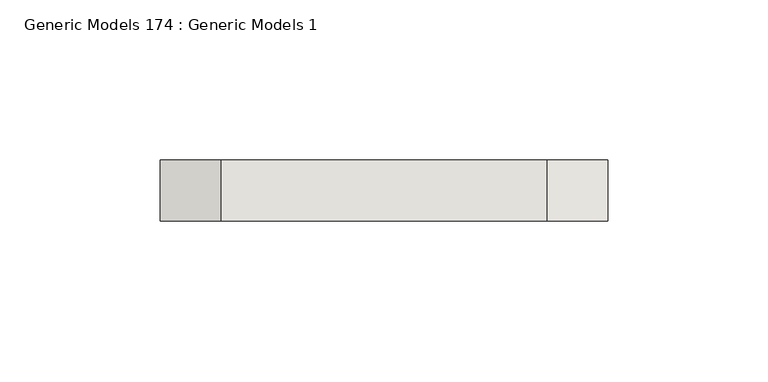
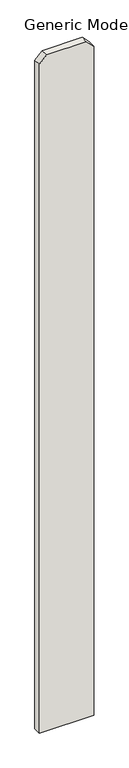
"""IFC4 building model written with IfcOpenShell, lengths in millimetres: wall geometry, Generic Models 174 : Generic Models 1."""

from ifc_helpers import new_model, si_unit, frame, origin, place, context, project, spatial, polyline, outline, extrude, source, transform, mapped, element, save


def generic_models_174_generic_models_1_8f357170(model_context):
    return source(origin(), model_context, "Body", "SweptSolid", [
        extrude(outline(polyline([(76.2, 325499.4125), (1885.95, 325499.4125), (1905.0, 325480.3625), (1905.0, 325378.7625), (1885.95, 325359.7125), (76.2, 325359.7125), (76.2, 325499.4125)])), frame((0.0, 547.6875, 0.0), z_axis=(0.0, 1.0, 0.0), x_axis=(0.0, 0.0, 1.0)), (0.0, 0.0, 1.0), 19.05),
    ])


if __name__ == "__main__":
    model = new_model("IFC4")
    model_context = context("Model", 3, world=origin())
    ifc_project = project(units=[si_unit("LENGTHUNIT", "METRE", prefix="MILLI")], contexts=[model_context])
    site = spatial("IfcSite", under=ifc_project)
    building = spatial("IfcBuilding", under=site)
    placement = place(None, origin())
    generic_models_174_generic_models_1_shape = generic_models_174_generic_models_1_8f357170(model_context)
    element("IfcWall", 1, ObjectType="Generic Models 174 : Generic Models 1", at=placement, inside=building, context=model_context, shape_type="MappedRepresentation", body=[
        mapped(generic_models_174_generic_models_1_shape, transform((0.0, 0.0, 0.0), x_axis=(1.0, 0.0, 0.0), y_axis=(0.0, 1.0, 0.0), z_axis=(0.0, 0.0, 1.0))),
    ])
    save(model, "model.ifc")

# Revit data of these elements
# Element 1 (IfcWall, "Generic Models 174 : Generic Models 1")
#   Materials on its faces: "VERTICAL 1X6 CEDAR PLANKS W/ CLEAR WOOD SEALER"
# Materials
#   "VERTICAL 1X6 CEDAR PLANKS W/ CLEAR WOOD SEALER": class "Wood", colour RGB 234 198 147, transparency 0, Description = "Pinus Echinata", Cost = 0
